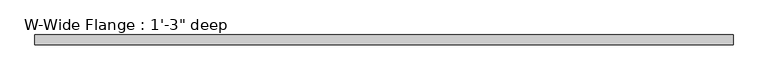
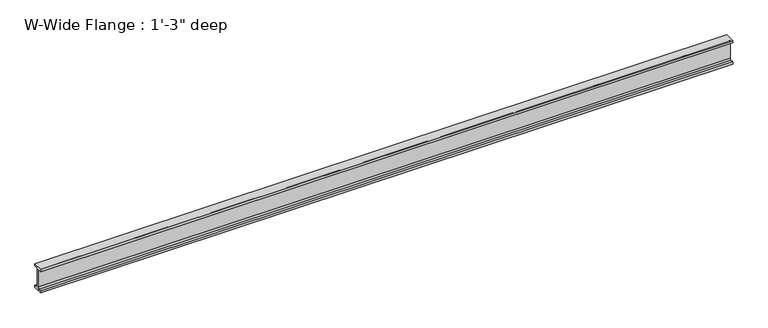
"""IFC4 building model written with IfcOpenShell, lengths in millimetres: beam geometry."""

from ifc_helpers import new_model, si_unit, point, frame, frame_2d, origin, place, context, project, spatial, polyline, circle_curve, trimmed, segment, composite_curve, outline, extrude, source, transform, mapped, element, save


def beam_34865ae6(model_context):
    return source(origin(), model_context, "Body", "SweptSolid", [
        extrude(outline(composite_curve([segment(polyline([(76.2, -155.956), (76.2, -190.5), (-76.2, -190.5), (-76.2, -155.956), (-32.131, -155.956)]), True, "CONTINUOUS"), segment(trimmed(circle_curve(frame_2d((-32.131, -133.35)), 22.606), [point((-32.131, -155.956))], [point((-9.525, -133.35))], True, "CARTESIAN"), True, "CONTINUOUS"), segment(polyline([(-9.525, -133.35), (-9.525, 133.35)]), True, "CONTINUOUS"), segment(trimmed(circle_curve(frame_2d((-32.131, 133.35)), 22.606), [point((-9.525, 133.35))], [point((-32.131, 155.956))], True, "CARTESIAN"), True, "CONTINUOUS"), segment(polyline([(-32.131, 155.956), (-76.2, 155.956), (-76.2, 190.5), (76.2, 190.5), (76.2, 155.956), (32.131, 155.956)]), True, "CONTINUOUS"), segment(trimmed(circle_curve(frame_2d((32.131, 133.35)), 22.606), [point((32.131, 155.956))], [point((9.525, 133.35))], True, "CARTESIAN"), True, "CONTINUOUS"), segment(polyline([(9.525, 133.35), (9.525, -133.35)]), True, "CONTINUOUS"), segment(trimmed(circle_curve(frame_2d((32.131, -133.35)), 22.606), [point((9.525, -133.35))], [point((32.131, -155.956))], True, "CARTESIAN"), True, "CONTINUOUS"), segment(polyline([(32.131, -155.956), (76.2, -155.956)]), True, "CONTINUOUS")], self_intersect=False)), frame((-5239.7019552, 0.0, 0.0), z_axis=(1.0, 0.0, 0.0), x_axis=(0.0, 1.0, 0.0)), (0.0, 0.0, 1.0), 10633.4516739),
    ])


if __name__ == "__main__":
    model = new_model("IFC4")
    model_context = context("Model", 3, world=origin())
    ifc_project = project(units=[si_unit("LENGTHUNIT", "METRE", prefix="MILLI")], contexts=[model_context])
    site = spatial("IfcSite", under=ifc_project)
    building = spatial("IfcBuilding", under=site)
    placement = place(None, origin())
    beam_shape = beam_34865ae6(model_context)
    element("IfcBeam", 1, ObjectType="W-Wide Flange : 1'-3\" deep", at=placement, inside=building, context=model_context, shape_type="MappedRepresentation", body=[
        mapped(beam_shape, transform((0.0, 0.0, 0.0), x_axis=(1.0, 0.0, 0.0), y_axis=(0.0, 1.0, 0.0), z_axis=(0.0, 0.0, 1.0))),
    ])
    save(model, "model.ifc")

# Revit data of these elements
# Type "W-Wide Flange : 1'-3\" deep"
#   Assembly Code = "B10"
#   W = 166
#   Length [instance default] = 5' - 0"
#   bf = 0' - 6"
#   d = 1' - 3"
#   k = 0' - 2 1/4"
#   k2 = 0' - 0.89"
#   tf = 0' - 1.36"
#   tw = 0' - 0 3/4"
#   A = 0.338889 SF
#   Structural Material [instance default] = Steel ASTM A992
# Element 1 (IfcBeam, "W-Wide Flange : 1'-3\" deep")
#   Structural Material = STRUCTURAL STEEL - SEE STRUCT. DWGS
#   Materials on its faces: "STRUCTURAL STEEL - SEE STRUCT. DWGS"
# Materials
#   "Steel ASTM A992": class "Metal", colour RGB 199 199 199, transparency 0, Description = "Structural steel 50ksi", Cost = 0
#   "STRUCTURAL STEEL - SEE STRUCT. DWGS": class "Metal", colour RGB 137 146 153, transparency 0, Description = "Steel, mill finish", Cost = 0
